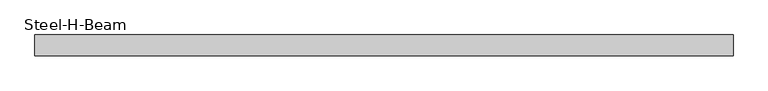
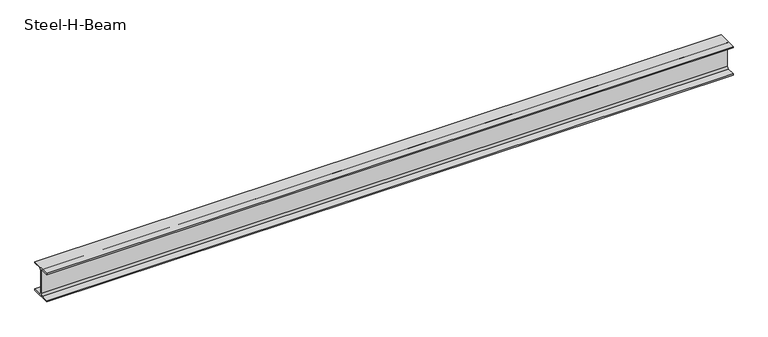
"""IFC4 building model written with IfcOpenShell, lengths in millimetres: beam geometry, Steel-H-Beam : BM121_H-294×200x8x12."""

import ifcopenshell
import ifcopenshell.guid

model = None  # the IFC model being written
_history = None  # IfcOwnerHistory: only IFC2X3 demands one
_inside = {}  # id of a spatial element -> (the spatial element, [elements in it])
_under = {}  # id of a project, library or spatial element -> (it, [spatial elements below it])
_declared = {}  # id of a project -> (the project, [libraries it declares])
_typed = {}  # id of a type object -> (the type object, [elements of that type])
_made_of = {}  # id of a material, layer set ... -> (it, [elements and type objects made of it])


def new_model(schema):
    """Start an empty IFC model of exactly this schema.

    Asked for "IFC4X3", IfcOpenShell would pick the latest addendum, in which some entities
    have other attributes; the version numbers below select the first issue.
    IFC2X3 requires an IfcOwnerHistory on every rooted entity: one is made here for all.
    """
    global model, _history
    if schema == "IFC4X3":
        model = ifcopenshell.file(schema_version=(4, 3, 0, 0))
    else:
        model = ifcopenshell.file(schema=schema)
    _inside.clear()
    _under.clear()
    _declared.clear()
    _typed.clear()
    _made_of.clear()
    _history = None
    if model.schema == "IFC2X3":
        org = make("IfcOrganization", Name="unknown")
        user = make(
            "IfcPersonAndOrganization",
            ThePerson=make("IfcPerson", FamilyName="unknown"),
            TheOrganization=org,
        )
        app = make(
            "IfcApplication",
            ApplicationDeveloper=org,
            Version="unknown",
            ApplicationFullName="unknown",
            ApplicationIdentifier="unknown",
        )
        _history = make(
            "IfcOwnerHistory",
            OwningUser=user,
            OwningApplication=app,
            ChangeAction="ADDED",
            CreationDate=0,
        )
    return model


def make(cls, **values):
    """One entity of the class cls with the attributes given. An attribute that is None is left unset."""
    return model.create_entity(
        cls, **{name: value for name, value in values.items() if value is not None}
    )


def rooted(cls, **values):
    """An entity with a GlobalId (a new one), such as an element, a storey or a relation."""
    return make(cls, GlobalId=ifcopenshell.guid.new(), OwnerHistory=_history, **values)


def si_unit(unit_type, name, prefix=None):
    """IfcSIUnit, for example si_unit("LENGTHUNIT", "METRE", prefix="MILLI")."""
    return make("IfcSIUnit", UnitType=unit_type, Prefix=prefix, Name=name)


def assignment(units):
    """IfcUnitAssignment: the units of a project."""
    return None if units is None else make("IfcUnitAssignment", Units=units)


def point(xyz):
    """IfcCartesianPoint."""
    return None if xyz is None else make("IfcCartesianPoint", Coordinates=xyz)


def direction(xyz):
    """IfcDirection."""
    return None if xyz is None else make("IfcDirection", DirectionRatios=xyz)


def frame(location, z_axis=None, x_axis=None):
    """IfcAxis2Placement3D, a coordinate frame: its origin and axes. An axis left out is left unset."""
    return make(
        "IfcAxis2Placement3D",
        Location=point(location),
        Axis=direction(z_axis),
        RefDirection=direction(x_axis),
    )


def frame_2d(location, x_axis=None):
    """IfcAxis2Placement2D, a coordinate frame in the plane: its origin and x axis."""
    return make(
        "IfcAxis2Placement2D", Location=point(location), RefDirection=direction(x_axis)
    )


def origin():
    """The frame at (0, 0, 0) with its axes left unset."""
    return frame((0.0, 0.0, 0.0))


def place(relative_to, where):
    """IfcLocalPlacement: puts the frame where relative to a parent placement (None: the world)."""
    return make(
        "IfcLocalPlacement", PlacementRelTo=relative_to, RelativePlacement=where
    )


def context(
    kind, dimensions, precision=None, world=None, true_north=None, identifier=None
):
    """IfcGeometricRepresentationContext, for example the 3D "Model" context."""
    return make(
        "IfcGeometricRepresentationContext",
        ContextIdentifier=identifier,
        ContextType=kind,
        CoordinateSpaceDimension=dimensions,
        Precision=precision,
        WorldCoordinateSystem=world,
        TrueNorth=true_north,
    )


def project(units=None, contexts=None):
    """IfcProject with its units and contexts."""
    return rooted(
        "IfcProject",
        Name="project",
        RepresentationContexts=contexts,
        UnitsInContext=assignment(units),
    )


def spatial(cls, under=None, at=None, **own):
    """A site, building, storey or space (cls), placed at a placement, below another one or the project."""
    s = rooted(cls, ObjectPlacement=at, **own)
    if under is not None:
        _under.setdefault(under.id(), (under, []))[1].append(s)
    return s


def polyline(points):
    """IfcPolyline through the points."""
    return make("IfcPolyline", Points=[point(p) for p in points])


def circle_curve(where, radius):
    """IfcCircle in the frame where."""
    return make("IfcCircle", Position=where, Radius=radius)


def trimmed(basis, trim1, trim2, sense, master):
    """IfcTrimmedCurve: the piece of a basis curve between two trims."""
    return make(
        "IfcTrimmedCurve",
        BasisCurve=basis,
        Trim1=trim1,
        Trim2=trim2,
        SenseAgreement=sense,
        MasterRepresentation=master,
    )


def segment(curve, same_sense, transition):
    """IfcCompositeCurveSegment."""
    return make(
        "IfcCompositeCurveSegment",
        Transition=transition,
        SameSense=same_sense,
        ParentCurve=curve,
    )


def composite_curve(segments, self_intersect=None):
    """IfcCompositeCurve: segments joined end to end."""
    return make("IfcCompositeCurve", Segments=segments, SelfIntersect=self_intersect)


def outline(outer, holes=None, kind="AREA"):
    """IfcArbitraryClosedProfileDef: a profile drawn as a closed curve; with holes, ...WithVoids."""
    if holes is None:
        return make("IfcArbitraryClosedProfileDef", ProfileType=kind, OuterCurve=outer)
    return make(
        "IfcArbitraryProfileDefWithVoids",
        ProfileType=kind,
        OuterCurve=outer,
        InnerCurves=holes,
    )


def extrude(swept, where, along, depth):
    """IfcExtrudedAreaSolid: the profile swept, set in the frame where, extruded along a direction by depth."""
    return make(
        "IfcExtrudedAreaSolid",
        SweptArea=swept,
        Position=where,
        ExtrudedDirection=direction(along),
        Depth=depth,
    )


def shape(context_of_items, identifier, shape_type, items):
    """IfcShapeRepresentation: the items that make up one representation, for example the "Body"."""
    return make(
        "IfcShapeRepresentation",
        ContextOfItems=context_of_items,
        RepresentationIdentifier=identifier,
        RepresentationType=shape_type,
        Items=items,
    )


def source(mapping_origin, context_of_items, identifier, shape_type, items):
    """IfcRepresentationMap: a shape defined once, which mapped items show again and again."""
    return make(
        "IfcRepresentationMap",
        MappingOrigin=mapping_origin,
        MappedRepresentation=shape(context_of_items, identifier, shape_type, items),
    )


def transform(
    local_origin,
    x_axis=None,
    y_axis=None,
    z_axis=None,
    scale=None,
    scale2=None,
    scale3=None,
    uniform=True,
):
    """IfcCartesianTransformationOperator3D, or its non-uniform kind. x_axis, y_axis, z_axis: its Axis1, 2, 3."""
    if uniform:
        return make(
            "IfcCartesianTransformationOperator3D",
            Axis1=direction(x_axis),
            Axis2=direction(y_axis),
            LocalOrigin=point(local_origin),
            Scale=scale,
            Axis3=direction(z_axis),
        )
    return make(
        "IfcCartesianTransformationOperator3DnonUniform",
        Axis1=direction(x_axis),
        Axis2=direction(y_axis),
        LocalOrigin=point(local_origin),
        Scale=scale,
        Axis3=direction(z_axis),
        Scale2=scale2,
        Scale3=scale3,
    )


def mapped(mapping_source, mapping_target):
    """IfcMappedItem: shows the shape of a source again, moved by a transform."""
    return make(
        "IfcMappedItem", MappingSource=mapping_source, MappingTarget=mapping_target
    )


def made_of(thing, what):
    """Note that an element or type object is made of a material, layer set ...; save() writes the relation."""
    if what is not None:
        _made_of.setdefault(what.id(), (what, []))[1].append(thing)
    return thing


def element(
    cls,
    number,
    at=None,
    inside=None,
    cuts=None,
    type_object=None,
    material=None,
    context=None,
    identifier="Body",
    shape_type=None,
    held_by="IfcProductDefinitionShape",
    body=None,
    shapes=None,
    **own,
):
    """One element of the class cls, such as IfcWall. Its Tag is "e" and its number.

    at: its placement. inside: the storey or other place that contains it. cuts: it is an
    opening in that element (IfcRelVoidsElement). A single representation is given by context,
    identifier, shape_type and body (its items); several are given by shapes. held_by: the class
    of the entity that holds the representations. save() writes the other relations.
    """
    e = rooted(cls, Tag="e%d" % number, ObjectPlacement=at, **own)
    if body is not None:
        shapes = [shape(context, identifier, shape_type, body)]
    if shapes is not None:
        e.Representation = make(held_by, Representations=shapes)
    if inside is not None:
        _inside.setdefault(inside.id(), (inside, []))[1].append(e)
    if cuts is not None:
        rooted(
            "IfcRelVoidsElement", RelatingBuildingElement=cuts, RelatedOpeningElement=e
        )
    if type_object is not None:
        _typed.setdefault(type_object.id(), (type_object, []))[1].append(e)
    return made_of(e, material)


def aggregate(whole, parts):
    """IfcRelAggregates: a whole, such as a stair, and the parts it consists of."""
    return rooted("IfcRelAggregates", RelatingObject=whole, RelatedObjects=parts)


def save(model, path):
    """Write the relations noted so far, then the file.

    IfcRelAggregates (storeys below a building ...), IfcRelContainedInSpatialStructure (elements
    in a storey), IfcRelDefinesByType, IfcRelAssociatesMaterial and IfcRelDeclares: one each for
    every whole, place, type object, material and project.
    """
    for whole, parts in _under.values():
        aggregate(whole, parts)
    for where, things in _inside.values():
        rooted(
            "IfcRelContainedInSpatialStructure",
            RelatedElements=things,
            RelatingStructure=where,
        )
    for kind, things in _typed.values():
        rooted("IfcRelDefinesByType", RelatedObjects=things, RelatingType=kind)
    for what, things in _made_of.values():
        rooted("IfcRelAssociatesMaterial", RelatedObjects=things, RelatingMaterial=what)
    for by, libraries in _declared.values():
        rooted("IfcRelDeclares", RelatingContext=by, RelatedDefinitions=libraries)
    model.write(path)


def steel_h_beam_f4173fa8(model_context):
    return source(origin(), model_context, "Body", "SweptSolid", [
        extrude(outline(composite_curve([segment(polyline([(100.0, -135.0), (100.0, -147.0), (-100.0, -147.0), (-100.0, -135.0), (-22.0, -135.0)]), True, "CONTINUOUS"), segment(trimmed(circle_curve(frame_2d((-22.0, -117.0)), 18.0), [point((-22.0, -135.0))], [point((-4.0, -117.0))], True, "CARTESIAN"), True, "CONTINUOUS"), segment(polyline([(-4.0, -117.0), (-4.0, 117.0)]), True, "CONTINUOUS"), segment(trimmed(circle_curve(frame_2d((-22.0, 117.0)), 18.0), [point((-4.0, 117.0))], [point((-22.0, 135.0))], True, "CARTESIAN"), True, "CONTINUOUS"), segment(polyline([(-22.0, 135.0), (-100.0, 135.0), (-100.0, 147.0), (100.0, 147.0), (100.0, 135.0), (22.0, 135.0)]), True, "CONTINUOUS"), segment(trimmed(circle_curve(frame_2d((22.0, 117.0)), 18.0), [point((22.0, 135.0))], [point((4.0, 117.0))], True, "CARTESIAN"), True, "CONTINUOUS"), segment(polyline([(4.0, 117.0), (4.0, -117.0)]), True, "CONTINUOUS"), segment(trimmed(circle_curve(frame_2d((22.0, -117.0)), 18.0), [point((4.0, -117.0))], [point((22.0, -135.0))], True, "CARTESIAN"), True, "CONTINUOUS"), segment(polyline([(22.0, -135.0), (100.0, -135.0)]), True, "CONTINUOUS")], self_intersect=False)), frame((-3361.3486745, 0.0, 0.0), z_axis=(1.0, 0.0, 0.0), x_axis=(0.0, 1.0, 0.0)), (0.0, 0.0, 1.0), 6724.6),
    ])


if __name__ == "__main__":
    model = new_model("IFC4")
    model_context = context("Model", 3, world=origin())
    ifc_project = project(units=[si_unit("LENGTHUNIT", "METRE", prefix="MILLI")], contexts=[model_context])
    site = spatial("IfcSite", under=ifc_project)
    building = spatial("IfcBuilding", under=site)
    placement = place(None, origin())
    steel_h_beam_shape = steel_h_beam_f4173fa8(model_context)
    element("IfcBeam", 1, ObjectType="Steel-H-Beam : BM121_H-294×200x8x12", at=placement, inside=building, context=model_context, shape_type="MappedRepresentation", body=[
        mapped(steel_h_beam_shape, transform((0.0, 0.0, 0.0), x_axis=(1.0, 0.0, 0.0), y_axis=(0.0, 1.0, 0.0), z_axis=(0.0, 0.0, 1.0))),
    ])
    save(model, "model.ifc")

# Revit data of these elements
# Type "Steel-H-Beam : BM121_H-294×200x8x12"
#   Surface Area = 1.3411 m²/m
#   Section Area = 72.3812 cm²
#   Mass per Unit Length = 56.8193 kg/m
#   Length [instance default] = 3000 mm
#   B = 200 mm
#   H = 294 mm
#   r = 18 mm
#   tw = 8 mm
#   tf = 12 mm
#   hec_material4 [instance default] = none
#   hec_material3 [instance default] = none
#   hec_material2 [instance default] = none
#   hec_material1 [instance default] = none
#   Structural Material [instance default] = Steel, 45-345
#   Assembly Code = ""
# Element 1 (IfcBeam, "Steel-H-Beam : BM121_H-294×200x8x12")
#   hec_material3 = F01AC000-00002_Building/Shelter Fire Proofing Work_Intumescent Coating Type_1 hr. rating (UL 1709))
#   hec_material2 = S01AA010-00002_Main Steel Structure Fabrication Work_Shelter/Building_Steel Painting/Coating_for Fireproofed Steel Surface, Surface Preparation & Primer Coat
#   hec_material1 = S03AA028-00001_Main Steel Structure Erection Work_Shelter/Building_Medium Steel
#   Structural Material = S01AA002-00001_Main Steel Structure Fabrication Work_Shelter/Building_Medium Steel - Standard
#   Materials on its faces: "S01AA002-00001_Main Steel Structure Fabrication Work_Shelter/Building_Medium Steel - Standard"
# Materials
#   "Steel, 45-345": class "Metal", colour RGB 189 187 185, transparency 0, Description = "Steel 345 MPa", Cost = 0
#   "S01AA002-00001_Main Steel Structure Fabrication Work_Shelter/Building_Medium Steel - Standard": class "Metal", colour RGB 120 120 120, transparency 0, Comments = "(90KG/M>Weight≥30KG/M)", Description = "Structural steel 50ksi", W00) Work Master Code = "S01AA002-0001", W01) Work Master_Lv1 = "Main Steel Structure Fabrication Work", W02) Work Master_Lv2 = "Shelter/Building", W03) Work Master_Spec.1 = "Medium Steel - Standard (90KG/M>Weight≥30KG/M)", Cost = 0
#   "F01AC000-00002_Building/Shelter Fire Proofing Work_Intumescent Coating Type_1 hr. rating (UL 1709))": class "Metal", colour RGB 255 128 128, transparency 0, Description = "Paint finished steel", W00) Work Master Code = "F01AC000-00002", W01) Work Master_Lv1 = "Building/Shelter Fire Proofing Work", W02) Work Master_Lv2 = "Intumescent Coating Type", W03) Work Master_Spec.1 = "1 hr. rating (UL 1709)", Cost = 0
#   "S01AA010-00002_Main Steel Structure Fabrication Work_Shelter/Building_Steel Painting/Coating_for Fireproofed Steel Surface, Surface Preparation & Primer Coat": class "Metal", colour RGB 120 120 120, transparency 0, Description = "Paint finished steel", W00) Work Master Code = "SS01AA010-00002", W01) Work Master_Lv1 = "Main Steel Structure Fabrication Work", W02) Work Master_Lv2 = "Shelter/Building", W03) Work Master_Spec.1 = "Steel Painting/Coating", W04) Work Master_Spec.2 = "for Fireproofed Steel Surface, Surface Preparation & Primer Coat", Cost = 0
#   "S03AA028-00001_Main Steel Structure Erection Work_Shelter/Building_Medium Steel": class "Metal", colour RGB 120 120 120, transparency 0, Comments = "(90KG/M>Weight≥30KG/M)", Description = "Structural steel 50ksi", W00) Work Master Code = "S03AA028-0001", W01) Work Master_Lv1 = "Main Steel Structure Erection Work", W02) Work Master_Lv2 = "Shelter/Building", W03) Work Master_Spec.1 = "Medium Steel (90KG/M>Weight≥30KG/M)", Cost = 0
